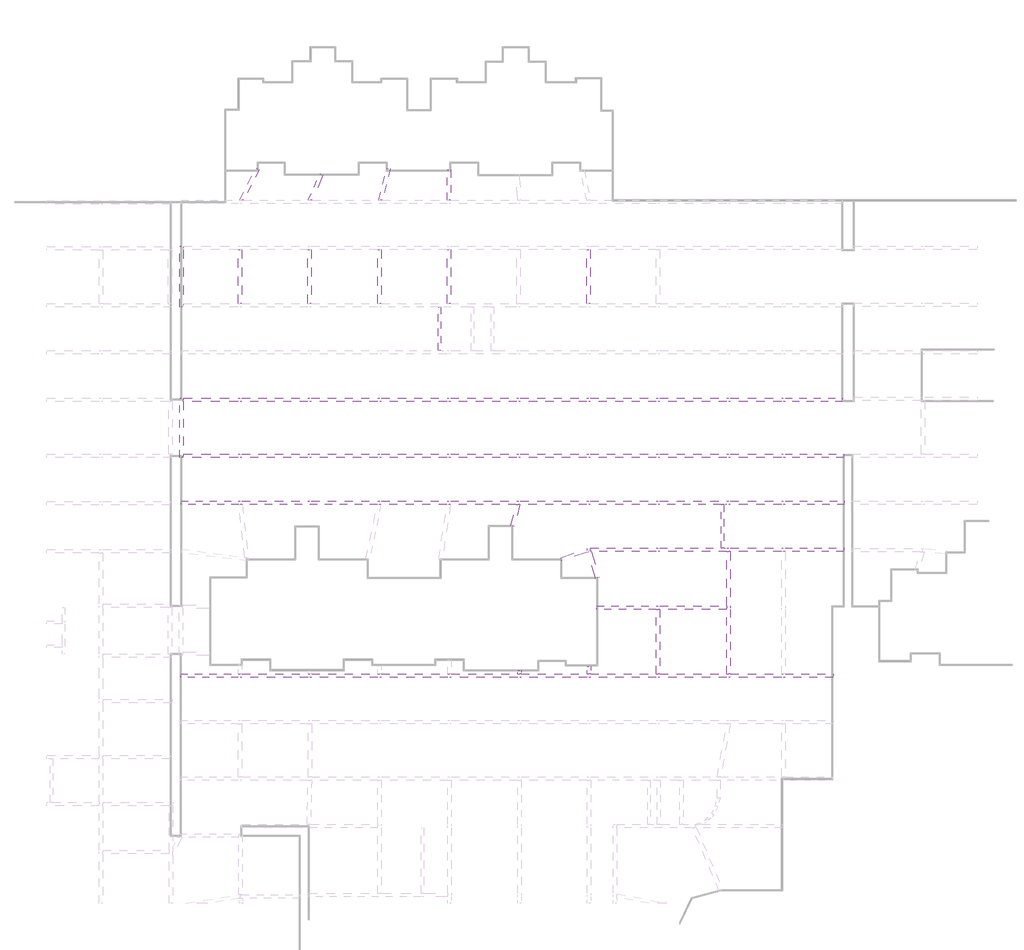
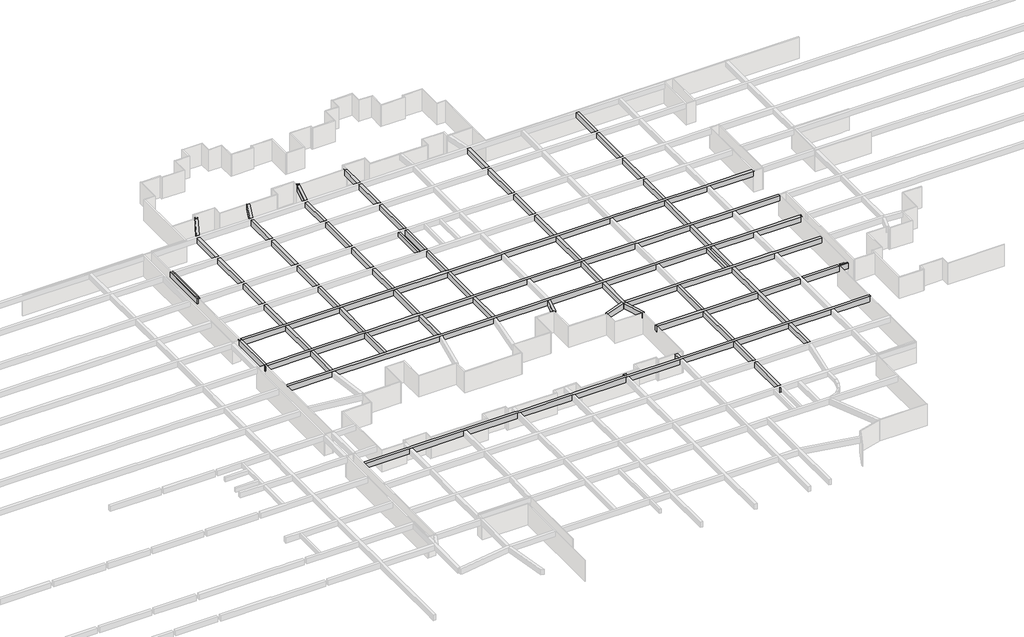
# One storey, part 13 of 16: 26 beams.
"""IFC4 building model written with IfcOpenShell, lengths in millimetres."""

from ifc_helpers import new_model, si_unit, frame, origin, place, context, project, spatial, polyline, outline, extrude, faceted_brep, element, save

model = new_model("IFC4")

# Units and contexts
model_context = context("Model", 3, world=origin())
ifc_project = project(units=[si_unit("LENGTHUNIT", "METRE", prefix="MILLI")], contexts=[model_context])

# Site, building, storey
site = spatial("IfcSite", under=ifc_project)
building = spatial("IfcBuilding", under=site)
storey = spatial("IfcBuildingStorey", under=building, Name="户型图", Elevation=0.0)

# Beams
placement = place(None, origin())
element("IfcBeam", 1, ObjectType="混凝土 - 矩形梁 : KL_beam", at=placement, inside=storey, context=model_context, shape_type="Brep", body=[
    faceted_brep([(256403.757676, -154958.1403142, 3300.0), (256003.757676, -154958.1403142, 3300.0), (256003.757676, -161826.0461868, 3300.0), (256403.757676, -161826.0461868, 3300.0), (256403.757676, -161426.0461868, 3300.0), (256403.757676, -155358.1403142, 3300.0), (256003.757676, -154958.1403142, 2500.0), (256003.757676, -161826.0461868, 2500.0), (256403.757676, -154958.1403142, 2500.0), (256403.757676, -155358.1403142, 2500.0), (256403.757676, -161426.0461868, 2500.0), (256403.757676, -161826.0461868, 2500.0)], [[[0, 1, 2, 3, 4, 5]], [[1, 6, 7, 2]], [[6, 8, 9, 10, 11, 7]], [[8, 0, 5, 4, 3, 11, 10, 9]], [[1, 0, 8, 6]], [[3, 2, 7, 11]]]),
])
element("IfcBeam", 2, ObjectType="混凝土 - 矩形梁 : KL_beam", at=placement, inside=storey, context=model_context, shape_type="Brep", body=[
    faceted_brep([(256403.757676, -137565.7214763, 3300.0), (256003.757676, -137565.7214763, 3300.0), (256003.757676, -144525.7214763, 3300.0), (256403.757676, -144525.7214763, 3300.0), (256403.757676, -144125.7214763, 3300.0), (256403.757676, -137965.7214763, 3300.0), (256403.757676, -137565.7214763, 2500.0), (256403.757676, -144525.7214763, 2500.0), (256403.757676, -144125.7214763, 2500.0), (256403.757676, -137965.7214763, 2500.0), (256003.757676, -137565.7214763, 2500.0), (256003.757676, -144525.7214763, 2500.0)], [[[0, 1, 2, 3, 4, 5]], [[6, 0, 5, 4, 3, 7, 8, 9]], [[10, 6, 9, 8, 7, 11]], [[1, 10, 11, 2]], [[1, 0, 6, 10]], [[3, 2, 11, 7]]]),
])
element("IfcBeam", 3, ObjectType="混凝土 - 矩形梁 : KL_beam", at=placement, inside=storey, context=model_context, shape_type="SweptSolid", body=[
    extrude(outline(polyline([(264780.5419955, -128606.5045486), (265136.9446052, -128788.1007485), (263349.1220942, -132296.8999905), (262900.1915992, -132296.8999905), (264780.5419955, -128606.5045486)])), frame((0.0, 0.0, 2500.0), z_axis=(0.0, 0.0, 1.0), x_axis=(1.0, 0.0, 0.0)), (0.0, 0.0, 1.0), 800.0),
])
element("IfcBeam", 4, ObjectType="混凝土 - 矩形梁 : KL_beam", at=placement, inside=storey, context=model_context, shape_type="SweptSolid", body=[
    extrude(outline(polyline([(272073.9960379, -129262.0850118), (272442.1979793, -129418.3774632), (271220.3376586, -132296.8999905), (270785.7935076, -132296.8999905), (272073.9960379, -129262.0850118)])), frame((0.0, 0.0, 2500.0), z_axis=(0.0, 0.0, 1.0), x_axis=(1.0, 0.0, 0.0)), (0.0, 0.0, 1.0), 800.0),
])
element("IfcBeam", 5, ObjectType="混凝土 - 矩形梁 : KL_beam", at=placement, inside=storey, context=model_context, shape_type="SweptSolid", body=[
    extrude(outline(polyline([(279764.8192397, -128598.9265902), (280152.9375302, -128695.6953484), (279255.0563689, -132296.8999905), (278842.8109172, -132296.8999905), (279764.8192397, -128598.9265902)])), frame((0.0, 0.0, 2500.0), z_axis=(0.0, 0.0, 1.0), x_axis=(1.0, 0.0, 0.0)), (0.0, 0.0, 1.0), 800.0),
])
element("IfcBeam", 6, ObjectType="混凝土 - 矩形梁 : KL_beam", at=placement, inside=storey, context=model_context, shape_type="SweptSolid", body=[
    extrude(outline(polyline([(286699.7203632, -128796.8999905), (287099.7203632, -128796.8999905), (287099.7203632, -132296.8999905), (286699.7203632, -132296.8999905), (286699.7203632, -128796.8999905)])), frame((0.0, 0.0, 2500.0), z_axis=(0.0, 0.0, 1.0), x_axis=(1.0, 0.0, 0.0)), (0.0, 0.0, 1.0), 800.0),
])
element("IfcBeam", 7, ObjectType="混凝土 - 矩形梁 : KL_beam", at=placement, inside=storey, context=model_context, shape_type="Brep", body=[
    faceted_brep([(332003.757676, -154958.1403142, 3300.0), (332003.757676, -155358.1403142, 3300.0), (332003.757676, -155358.1403142, 2500.0), (332003.757676, -154958.1403142, 2500.0), (325452.9173169, -154958.1403142, 3300.0), (325052.9173169, -154958.1403142, 3300.0), (319175.2880408, -154958.1403142, 3300.0), (318775.2880408, -154958.1403142, 3300.0), (311075.2880408, -154958.1403142, 3300.0), (310675.2880408, -154958.1403142, 3300.0), (303119.0558962, -154958.1403142, 3300.0), (302719.0558962, -154958.1403142, 3300.0), (295091.573786, -154958.1403142, 3300.0), (294691.573786, -154958.1403142, 3300.0), (287099.7203632, -154958.1403142, 3300.0), (286699.7203632, -154958.1403142, 3300.0), (279139.6845219, -154958.1403142, 3300.0), (278739.6845219, -154958.1403142, 3300.0), (271118.1706199, -154958.1403142, 3300.0), (270718.1706199, -154958.1403142, 3300.0), (263155.329592, -154958.1403142, 3300.0), (262755.329592, -154958.1403142, 3300.0), (256403.757676, -154958.1403142, 3300.0), (256403.757676, -155358.1403142, 3300.0), (262755.329592, -155358.1403142, 3300.0), (263155.329592, -155358.1403142, 3300.0), (270718.1706199, -155358.1403142, 3300.0), (271118.1706199, -155358.1403142, 3300.0), (278739.6845219, -155358.1403142, 3300.0), (279139.6845219, -155358.1403142, 3300.0), (286699.7203632, -155358.1403142, 3300.0), (287099.7203632, -155358.1403142, 3300.0), (294691.573786, -155358.1403142, 3300.0), (295091.573786, -155358.1403142, 3300.0), (302719.0558962, -155358.1403142, 3300.0), (303119.0558962, -155358.1403142, 3300.0), (310675.2880408, -155358.1403142, 3300.0), (311075.2880408, -155358.1403142, 3300.0), (318775.2880408, -155358.1403142, 3300.0), (319175.2880408, -155358.1403142, 3300.0), (325052.9173169, -155358.1403142, 3300.0), (325452.9173169, -155358.1403142, 3300.0), (256403.757676, -155358.1403142, 2500.0), (262755.329592, -155358.1403142, 2500.0), (263155.329592, -155358.1403142, 2500.0), (270718.1706199, -155358.1403142, 2500.0), (271118.1706199, -155358.1403142, 2500.0), (278739.6845219, -155358.1403142, 2500.0), (279139.6845219, -155358.1403142, 2500.0), (286699.7203632, -155358.1403142, 2500.0), (287099.7203632, -155358.1403142, 2500.0), (294691.573786, -155358.1403142, 2500.0), (295091.573786, -155358.1403142, 2500.0), (302719.0558962, -155358.1403142, 2500.0), (303119.0558962, -155358.1403142, 2500.0), (310675.2880408, -155358.1403142, 2500.0), (311075.2880408, -155358.1403142, 2500.0), (318775.2880408, -155358.1403142, 2500.0), (319175.2880408, -155358.1403142, 2500.0), (325052.9173169, -155358.1403142, 2500.0), (325452.9173169, -155358.1403142, 2500.0), (256403.757676, -154958.1403142, 2500.0), (262755.329592, -154958.1403142, 2500.0), (263155.329592, -154958.1403142, 2500.0), (270718.1706199, -154958.1403142, 2500.0), (271118.1706199, -154958.1403142, 2500.0), (278739.6845219, -154958.1403142, 2500.0), (279139.6845219, -154958.1403142, 2500.0), (286699.7203632, -154958.1403142, 2500.0), (287099.7203632, -154958.1403142, 2500.0), (294691.573786, -154958.1403142, 2500.0), (295091.573786, -154958.1403142, 2500.0), (302719.0558962, -154958.1403142, 2500.0), (303119.0558962, -154958.1403142, 2500.0), (310675.2880408, -154958.1403142, 2500.0), (311075.2880408, -154958.1403142, 2500.0), (318775.2880408, -154958.1403142, 2500.0), (319175.2880408, -154958.1403142, 2500.0), (325052.9173169, -154958.1403142, 2500.0), (325452.9173169, -154958.1403142, 2500.0)], [[[0, 1, 2, 3]], [[1, 0, 4, 5, 6, 7, 8, 9, 10, 11, 12, 13, 14, 15, 16, 17, 18, 19, 20, 21, 22, 23, 24, 25, 26, 27, 28, 29, 30, 31, 32, 33, 34, 35, 36, 37, 38, 39, 40, 41]], [[2, 1, 41, 40, 39, 38, 37, 36, 35, 34, 33, 32, 31, 30, 29, 28, 27, 26, 25, 24, 23, 42, 43, 44, 45, 46, 47, 48, 49, 50, 51, 52, 53, 54, 55, 56, 57, 58, 59, 60]], [[3, 2, 60, 59, 58, 57, 56, 55, 54, 53, 52, 51, 50, 49, 48, 47, 46, 45, 44, 43, 42, 61, 62, 63, 64, 65, 66, 67, 68, 69, 70, 71, 72, 73, 74, 75, 76, 77, 78, 79]], [[0, 3, 79, 78, 77, 76, 75, 74, 73, 72, 71, 70, 69, 68, 67, 66, 65, 64, 63, 62, 61, 22, 21, 20, 19, 18, 17, 16, 15, 14, 13, 12, 11, 10, 9, 8, 7, 6, 5, 4]], [[23, 22, 61, 42]]]),
])
element("IfcBeam", 8, ObjectType="混凝土 - 矩形梁 : KL_beam", at=placement, inside=storey, context=model_context, shape_type="Brep", body=[
    faceted_brep([(332153.7576761, -161426.0461868, 3300.0), (332153.7576761, -161826.0461868, 3300.0), (332153.7576761, -161826.0461868, 2500.0), (332153.7576761, -161426.0461868, 2500.0), (325452.9173169, -161426.0461868, 3300.0), (325052.9173169, -161426.0461868, 3300.0), (319175.2880408, -161426.0461868, 3300.0), (318775.2880408, -161426.0461868, 3300.0), (311075.2880408, -161426.0461868, 3300.0), (310675.2880408, -161426.0461868, 3300.0), (303119.0558962, -161426.0461868, 3300.0), (302719.0558962, -161426.0461868, 3300.0), (295091.573786, -161426.0461868, 3300.0), (294691.573786, -161426.0461868, 3300.0), (287099.7203632, -161426.0461868, 3300.0), (286699.7203632, -161426.0461868, 3300.0), (279139.6845219, -161426.0461868, 3300.0), (278739.6845219, -161426.0461868, 3300.0), (271118.1706199, -161426.0461868, 3300.0), (270718.1706199, -161426.0461868, 3300.0), (263155.329592, -161426.0461868, 3300.0), (262755.329592, -161426.0461868, 3300.0), (256403.757676, -161426.0461868, 3300.0), (256403.757676, -161826.0461868, 3300.0), (262755.329592, -161826.0461868, 3300.0), (263155.329592, -161826.0461868, 3300.0), (270718.1706199, -161826.0461868, 3300.0), (271118.1706199, -161826.0461868, 3300.0), (278739.6845219, -161826.0461868, 3300.0), (279139.6845219, -161826.0461868, 3300.0), (286699.7203632, -161826.0461868, 3300.0), (287099.7203632, -161826.0461868, 3300.0), (294691.573786, -161826.0461868, 3300.0), (295091.573786, -161826.0461868, 3300.0), (302719.0558962, -161826.0461868, 3300.0), (303119.0558962, -161826.0461868, 3300.0), (310675.2880408, -161826.0461868, 3300.0), (311075.2880408, -161826.0461868, 3300.0), (318775.2880408, -161826.0461868, 3300.0), (319175.2880408, -161826.0461868, 3300.0), (325052.9173169, -161826.0461868, 3300.0), (325452.9173169, -161826.0461868, 3300.0), (256403.757676, -161826.0461868, 2500.0), (262755.329592, -161826.0461868, 2500.0), (263155.329592, -161826.0461868, 2500.0), (270718.1706199, -161826.0461868, 2500.0), (271118.1706199, -161826.0461868, 2500.0), (278739.6845219, -161826.0461868, 2500.0), (279139.6845219, -161826.0461868, 2500.0), (286699.7203632, -161826.0461868, 2500.0), (287099.7203632, -161826.0461868, 2500.0), (294691.573786, -161826.0461868, 2500.0), (295091.573786, -161826.0461868, 2500.0), (302719.0558962, -161826.0461868, 2500.0), (303119.0558962, -161826.0461868, 2500.0), (310675.2880408, -161826.0461868, 2500.0), (311075.2880408, -161826.0461868, 2500.0), (318775.2880408, -161826.0461868, 2500.0), (319175.2880408, -161826.0461868, 2500.0), (325052.9173169, -161826.0461868, 2500.0), (325452.9173169, -161826.0461868, 2500.0), (256403.757676, -161426.0461868, 2500.0), (262755.329592, -161426.0461868, 2500.0), (263155.329592, -161426.0461868, 2500.0), (270718.1706199, -161426.0461868, 2500.0), (271118.1706199, -161426.0461868, 2500.0), (278739.6845219, -161426.0461868, 2500.0), (279139.6845219, -161426.0461868, 2500.0), (286699.7203632, -161426.0461868, 2500.0), (287099.7203632, -161426.0461868, 2500.0), (294691.573786, -161426.0461868, 2500.0), (295091.573786, -161426.0461868, 2500.0), (302719.0558962, -161426.0461868, 2500.0), (303119.0558962, -161426.0461868, 2500.0), (310675.2880408, -161426.0461868, 2500.0), (311075.2880408, -161426.0461868, 2500.0), (318775.2880408, -161426.0461868, 2500.0), (319175.2880408, -161426.0461868, 2500.0), (325052.9173169, -161426.0461868, 2500.0), (325452.9173169, -161426.0461868, 2500.0)], [[[0, 1, 2, 3]], [[1, 0, 4, 5, 6, 7, 8, 9, 10, 11, 12, 13, 14, 15, 16, 17, 18, 19, 20, 21, 22, 23, 24, 25, 26, 27, 28, 29, 30, 31, 32, 33, 34, 35, 36, 37, 38, 39, 40, 41]], [[2, 1, 41, 40, 39, 38, 37, 36, 35, 34, 33, 32, 31, 30, 29, 28, 27, 26, 25, 24, 23, 42, 43, 44, 45, 46, 47, 48, 49, 50, 51, 52, 53, 54, 55, 56, 57, 58, 59, 60]], [[3, 2, 60, 59, 58, 57, 56, 55, 54, 53, 52, 51, 50, 49, 48, 47, 46, 45, 44, 43, 42, 61, 62, 63, 64, 65, 66, 67, 68, 69, 70, 71, 72, 73, 74, 75, 76, 77, 78, 79]], [[0, 3, 79, 78, 77, 76, 75, 74, 73, 72, 71, 70, 69, 68, 67, 66, 65, 64, 63, 62, 61, 22, 21, 20, 19, 18, 17, 16, 15, 14, 13, 12, 11, 10, 9, 8, 7, 6, 5, 4]], [[23, 22, 61, 42]]]),
])
element("IfcBeam", 9, ObjectType="混凝土 - 矩形梁 : KL_beam", at=placement, inside=storey, context=model_context, shape_type="Brep", body=[
    faceted_brep([(332253.7576761, -166823.3600959, 3300.0), (332253.7576761, -167223.3600959, 3300.0), (332253.7576761, -167223.3600959, 2500.0), (332253.7576761, -166823.3600959, 2500.0), (256203.7576761, -166823.3600959, 3300.0), (256203.7576761, -166823.3600959, 2500.0), (256203.7576761, -167223.3600959, 2500.0), (256203.7576761, -167223.3600959, 3300.0), (325452.9173169, -166823.3600959, 3300.0), (325052.9173169, -166823.3600959, 3300.0), (319175.2880408, -166823.3600959, 3300.0), (318775.2880408, -166823.3600959, 3300.0), (311075.2880408, -166823.3600959, 3300.0), (310675.2880408, -166823.3600959, 3300.0), (303119.0558962, -166823.3600959, 3300.0), (302719.0558962, -166823.3600959, 3300.0), (295091.573786, -166823.3600959, 3300.0), (294691.573786, -166823.3600959, 3300.0), (287099.7203632, -166823.3600959, 3300.0), (286699.7203632, -166823.3600959, 3300.0), (279139.6845219, -166823.3600959, 3300.0), (278739.6845219, -166823.3600959, 3300.0), (271118.1706199, -166823.3600959, 3300.0), (270718.1706199, -166823.3600959, 3300.0), (263155.329592, -166823.3600959, 3300.0), (262755.329592, -166823.3600959, 3300.0), (262777.848794, -167223.3600959, 3300.0), (263180.706086, -167223.3600959, 3300.0), (278692.7050906, -167223.3600959, 3300.0), (279101.6413286, -167223.3600959, 3300.0), (286667.5284745, -167223.3600959, 3300.0), (287071.9916696, -167223.3600959, 3300.0), (294630.9287114, -167223.3600959, 3300.0), (295045.0391836, -167223.3600959, 3300.0), (302719.0558962, -167223.3600959, 3300.0), (303119.0558962, -167223.3600959, 3300.0), (310675.2880408, -167223.3600959, 3300.0), (311075.2880408, -167223.3600959, 3300.0), (318103.757676, -167223.3600959, 3300.0), (318403.757676, -167223.3600959, 3300.0), (318775.2880408, -167223.3600959, 3300.0), (319175.2880408, -167223.3600959, 3300.0), (325052.9173169, -167223.3600959, 3300.0), (325452.9173169, -167223.3600959, 3300.0), (262777.848794, -167223.3600959, 2500.0), (263180.706086, -167223.3600959, 2500.0), (278692.7050906, -167223.3600959, 2500.0), (279101.6413286, -167223.3600959, 2500.0), (286667.5284745, -167223.3600959, 2500.0), (287071.9916696, -167223.3600959, 2500.0), (294630.9287114, -167223.3600959, 2500.0), (295045.0391836, -167223.3600959, 2500.0), (302719.0558962, -167223.3600959, 2500.0), (303119.0558962, -167223.3600959, 2500.0), (310675.2880408, -167223.3600959, 2500.0), (311075.2880408, -167223.3600959, 2500.0), (318775.2880408, -167223.3600959, 2500.0), (319175.2880408, -167223.3600959, 2500.0), (325052.9173169, -167223.3600959, 2500.0), (325452.9173169, -167223.3600959, 2500.0), (262755.329592, -166823.3600959, 2500.0), (263155.329592, -166823.3600959, 2500.0), (270718.1706199, -166823.3600959, 2500.0), (271118.1706199, -166823.3600959, 2500.0), (278739.6845219, -166823.3600959, 2500.0), (279139.6845219, -166823.3600959, 2500.0), (286699.7203632, -166823.3600959, 2500.0), (287099.7203632, -166823.3600959, 2500.0), (294691.573786, -166823.3600959, 2500.0), (295091.573786, -166823.3600959, 2500.0), (302719.0558962, -166823.3600959, 2500.0), (303119.0558962, -166823.3600959, 2500.0), (310675.2880408, -166823.3600959, 2500.0), (311075.2880408, -166823.3600959, 2500.0), (318775.2880408, -166823.3600959, 2500.0), (319175.2880408, -166823.3600959, 2500.0), (325052.9173169, -166823.3600959, 2500.0), (325452.9173169, -166823.3600959, 2500.0)], [[[0, 1, 2, 3]], [[4, 5, 6, 7]], [[1, 0, 8, 9, 10, 11, 12, 13, 14, 15, 16, 17, 18, 19, 20, 21, 22, 23, 24, 25, 4, 7, 26, 27, 28, 29, 30, 31, 32, 33, 34, 35, 36, 37, 38, 39, 40, 41, 42, 43]], [[2, 1, 43, 42, 41, 40, 39, 38, 37, 36, 35, 34, 33, 32, 31, 30, 29, 28, 27, 26, 7, 6, 44, 45, 46, 47, 48, 49, 50, 51, 52, 53, 54, 55, 56, 57, 58, 59]], [[3, 2, 59, 58, 57, 56, 55, 54, 53, 52, 51, 50, 49, 48, 47, 46, 45, 44, 6, 5, 60, 61, 62, 63, 64, 65, 66, 67, 68, 69, 70, 71, 72, 73, 74, 75, 76, 77]], [[0, 3, 77, 76, 75, 74, 73, 72, 71, 70, 69, 68, 67, 66, 65, 64, 63, 62, 61, 60, 5, 4, 25, 24, 23, 22, 21, 20, 19, 18, 17, 16, 15, 14, 13, 12, 11, 10, 9, 8]]]),
])
element("IfcBeam", 10, ObjectType="混凝土 - 矩形梁 : KL_beam", at=placement, inside=storey, context=model_context, shape_type="Brep", body=[
    faceted_brep([(330953.597965, -186662.1668684, 3300.0), (330953.597965, -187062.1668684, 3300.0), (330953.597965, -187062.1668684, 2500.0), (330953.597965, -186662.1668684, 2500.0), (256118.597965, -186662.1668684, 3300.0), (256118.597965, -186662.1668684, 2500.0), (256118.597965, -187062.1668684, 2500.0), (256118.597965, -187062.1668684, 3300.0), (325452.9173169, -186662.1668684, 3300.0), (325052.9173169, -186662.1668684, 3300.0), (319175.2880408, -186662.1668684, 3300.0), (318775.2880408, -186662.1668684, 3300.0), (311075.2880408, -186662.1668684, 3300.0), (310675.2880408, -186662.1668684, 3300.0), (303155.2880408, -186662.1668684, 3300.0), (302755.2880408, -186662.1668684, 3300.0), (295188.9093069, -186662.1668684, 3300.0), (294788.9093069, -186662.1668684, 3300.0), (287188.9093069, -186662.1668684, 3300.0), (286788.9093069, -186662.1668684, 3300.0), (279139.4840766, -186662.1668684, 3300.0), (278739.4840766, -186662.1668684, 3300.0), (271154.6470805, -186662.1668684, 3300.0), (270754.6470805, -186662.1668684, 3300.0), (263153.757676, -186662.1668684, 3300.0), (262753.757676, -186662.1668684, 3300.0), (262753.757676, -187062.1668684, 3300.0), (263153.757676, -187062.1668684, 3300.0), (270754.6470805, -187062.1668684, 3300.0), (271154.6470805, -187062.1668684, 3300.0), (278739.4840766, -187062.1668684, 3300.0), (279139.4840766, -187062.1668684, 3300.0), (286788.9093069, -187062.1668684, 3300.0), (287188.9093069, -187062.1668684, 3300.0), (294788.9093069, -187062.1668684, 3300.0), (295188.9093069, -187062.1668684, 3300.0), (302755.2880408, -187062.1668684, 3300.0), (303155.2880408, -187062.1668684, 3300.0), (310675.2880408, -187062.1668684, 3300.0), (311075.2880408, -187062.1668684, 3300.0), (318775.2880408, -187062.1668684, 3300.0), (319175.2880408, -187062.1668684, 3300.0), (325052.9173169, -187062.1668684, 3300.0), (325452.9173169, -187062.1668684, 3300.0), (262753.757676, -187062.1668684, 2500.0), (263153.757676, -187062.1668684, 2500.0), (270754.6470805, -187062.1668684, 2500.0), (271154.6470805, -187062.1668684, 2500.0), (278739.4840766, -187062.1668684, 2500.0), (279139.4840766, -187062.1668684, 2500.0), (286788.9093069, -187062.1668684, 2500.0), (287188.9093069, -187062.1668684, 2500.0), (294788.9093069, -187062.1668684, 2500.0), (295188.9093069, -187062.1668684, 2500.0), (302755.2880408, -187062.1668684, 2500.0), (303155.2880408, -187062.1668684, 2500.0), (310675.2880408, -187062.1668684, 2500.0), (311075.2880408, -187062.1668684, 2500.0), (318775.2880408, -187062.1668684, 2500.0), (319175.2880408, -187062.1668684, 2500.0), (325052.9173169, -187062.1668684, 2500.0), (325452.9173169, -187062.1668684, 2500.0), (262753.757676, -186662.1668684, 2500.0), (263153.757676, -186662.1668684, 2500.0), (270754.6470805, -186662.1668684, 2500.0), (271154.6470805, -186662.1668684, 2500.0), (278739.4840766, -186662.1668684, 2500.0), (279139.4840766, -186662.1668684, 2500.0), (286788.9093069, -186662.1668684, 2500.0), (287188.9093069, -186662.1668684, 2500.0), (294788.9093069, -186662.1668684, 2500.0), (295188.9093069, -186662.1668684, 2500.0), (302755.2880408, -186662.1668684, 2500.0), (303155.2880408, -186662.1668684, 2500.0), (310675.2880408, -186662.1668684, 2500.0), (311075.2880408, -186662.1668684, 2500.0), (318775.2880408, -186662.1668684, 2500.0), (319175.2880408, -186662.1668684, 2500.0), (325052.9173169, -186662.1668684, 2500.0), (325452.9173169, -186662.1668684, 2500.0)], [[[0, 1, 2, 3]], [[4, 5, 6, 7]], [[1, 0, 8, 9, 10, 11, 12, 13, 14, 15, 16, 17, 18, 19, 20, 21, 22, 23, 24, 25, 4, 7, 26, 27, 28, 29, 30, 31, 32, 33, 34, 35, 36, 37, 38, 39, 40, 41, 42, 43]], [[2, 1, 43, 42, 41, 40, 39, 38, 37, 36, 35, 34, 33, 32, 31, 30, 29, 28, 27, 26, 7, 6, 44, 45, 46, 47, 48, 49, 50, 51, 52, 53, 54, 55, 56, 57, 58, 59, 60, 61]], [[3, 2, 61, 60, 59, 58, 57, 56, 55, 54, 53, 52, 51, 50, 49, 48, 47, 46, 45, 44, 6, 5, 62, 63, 64, 65, 66, 67, 68, 69, 70, 71, 72, 73, 74, 75, 76, 77, 78, 79]], [[0, 3, 79, 78, 77, 76, 75, 74, 73, 72, 71, 70, 69, 68, 67, 66, 65, 64, 63, 62, 5, 4, 25, 24, 23, 22, 21, 20, 19, 18, 17, 16, 15, 14, 13, 12, 11, 10, 9, 8]]]),
])
element("IfcBeam", 11, ObjectType="混凝土 - 矩形梁 : KL_beam", at=placement, inside=storey, context=model_context, shape_type="SweptSolid", body=[
    extrude(outline(polyline([(302755.2880408, -185762.1668684), (303155.2880408, -185762.1668684), (303155.2880408, -186662.1668684), (302755.2880408, -186662.1668684), (302755.2880408, -185762.1668684)])), frame((0.0, 0.0, 2500.0), z_axis=(0.0, 0.0, 1.0), x_axis=(1.0, 0.0, 0.0)), (0.0, 0.0, 1.0), 800.0),
])
element("IfcBeam", 12, ObjectType="混凝土 - 矩形梁 : KL_beam", at=placement, inside=storey, context=model_context, shape_type="SweptSolid", body=[
    extrude(outline(polyline([(294788.9093069, -186227.0533069), (295188.9093069, -186227.0533069), (295188.9093069, -186662.1668684), (294788.9093069, -186662.1668684), (294788.9093069, -186227.0533069)])), frame((0.0, 0.0, 2500.0), z_axis=(0.0, 0.0, 1.0), x_axis=(1.0, 0.0, 0.0)), (0.0, 0.0, 1.0), 800.0),
])
element("IfcBeam", 13, ObjectType="混凝土 - 矩形梁 : KL_beam", at=placement, inside=storey, context=model_context, shape_type="SweptSolid", body=[
    extrude(outline(polyline([(263155.329592, -166823.3600959), (262755.329592, -166823.3600959), (262755.329592, -161826.0461868), (263155.329592, -161826.0461868), (263155.329592, -166823.3600959)])), frame((0.0, 0.0, 2500.0), z_axis=(0.0, 0.0, 1.0), x_axis=(1.0, 0.0, 0.0)), (0.0, 0.0, 1.0), 800.0),
    extrude(outline(polyline([(262755.329592, -132696.8999905), (263155.329592, -132696.8999905), (263155.329592, -137565.7214763), (262755.329592, -137565.7214763), (262755.329592, -132696.8999905)])), frame((0.0, 0.0, 2500.0), z_axis=(0.0, 0.0, 1.0), x_axis=(1.0, 0.0, 0.0)), (0.0, 0.0, 1.0), 800.0),
    extrude(outline(polyline([(262755.329592, -137965.7214763), (263155.329592, -137965.7214763), (263155.329592, -144125.7214763), (262755.329592, -144125.7214763), (262755.329592, -137965.7214763)])), frame((0.0, 0.0, 2500.0), z_axis=(0.0, 0.0, 1.0), x_axis=(1.0, 0.0, 0.0)), (0.0, 0.0, 1.0), 800.0),
    extrude(outline(polyline([(262755.329592, -144525.7214763), (263155.329592, -144525.7214763), (263155.329592, -149525.7214763), (262755.329592, -149525.7214763), (262755.329592, -144525.7214763)])), frame((0.0, 0.0, 2500.0), z_axis=(0.0, 0.0, 1.0), x_axis=(1.0, 0.0, 0.0)), (0.0, 0.0, 1.0), 800.0),
    extrude(outline(polyline([(262755.329592, -149925.7214763), (263155.329592, -149925.7214763), (263155.329592, -154958.1403142), (262755.329592, -154958.1403142), (262755.329592, -149925.7214763)])), frame((0.0, 0.0, 2500.0), z_axis=(0.0, 0.0, 1.0), x_axis=(1.0, 0.0, 0.0)), (0.0, 0.0, 1.0), 800.0),
    extrude(outline(polyline([(262755.329592, -155358.1403142), (263155.329592, -155358.1403142), (263155.329592, -161426.0461868), (262755.329592, -161426.0461868), (262755.329592, -155358.1403142)])), frame((0.0, 0.0, 2500.0), z_axis=(0.0, 0.0, 1.0), x_axis=(1.0, 0.0, 0.0)), (0.0, 0.0, 1.0), 800.0),
])
element("IfcBeam", 14, ObjectType="混凝土 - 矩形梁 : KL_beam", at=placement, inside=storey, context=model_context, shape_type="SweptSolid", body=[
    extrude(outline(polyline([(270718.1706199, -132696.8999905), (271118.1706199, -132696.8999905), (271118.1706199, -137565.7214763), (270718.1706199, -137565.7214763), (270718.1706199, -132696.8999905)])), frame((0.0, 0.0, 2500.0), z_axis=(0.0, 0.0, 1.0), x_axis=(1.0, 0.0, 0.0)), (0.0, 0.0, 1.0), 800.0),
    extrude(outline(polyline([(271118.1706199, -166823.3600959), (270718.1706199, -166823.3600959), (270718.1706199, -161826.0461868), (271118.1706199, -161826.0461868), (271118.1706199, -166823.3600959)])), frame((0.0, 0.0, 2500.0), z_axis=(0.0, 0.0, 1.0), x_axis=(1.0, 0.0, 0.0)), (0.0, 0.0, 1.0), 800.0),
    extrude(outline(polyline([(270718.1706199, -137965.7214763), (271118.1706199, -137965.7214763), (271118.1706199, -144125.7214763), (270718.1706199, -144125.7214763), (270718.1706199, -137965.7214763)])), frame((0.0, 0.0, 2500.0), z_axis=(0.0, 0.0, 1.0), x_axis=(1.0, 0.0, 0.0)), (0.0, 0.0, 1.0), 800.0),
    extrude(outline(polyline([(270718.1706199, -144525.7214763), (271118.1706199, -144525.7214763), (271118.1706199, -149525.7214763), (270718.1706199, -149525.7214763), (270718.1706199, -144525.7214763)])), frame((0.0, 0.0, 2500.0), z_axis=(0.0, 0.0, 1.0), x_axis=(1.0, 0.0, 0.0)), (0.0, 0.0, 1.0), 800.0),
    extrude(outline(polyline([(270718.1706199, -149925.7214763), (271118.1706199, -149925.7214763), (271118.1706199, -154958.1403142), (270718.1706199, -154958.1403142), (270718.1706199, -149925.7214763)])), frame((0.0, 0.0, 2500.0), z_axis=(0.0, 0.0, 1.0), x_axis=(1.0, 0.0, 0.0)), (0.0, 0.0, 1.0), 800.0),
    extrude(outline(polyline([(270718.1706199, -155358.1403142), (271118.1706199, -155358.1403142), (271118.1706199, -161426.0461868), (270718.1706199, -161426.0461868), (270718.1706199, -155358.1403142)])), frame((0.0, 0.0, 2500.0), z_axis=(0.0, 0.0, 1.0), x_axis=(1.0, 0.0, 0.0)), (0.0, 0.0, 1.0), 800.0),
])
element("IfcBeam", 15, ObjectType="混凝土 - 矩形梁 : KL_beam", at=placement, inside=storey, context=model_context, shape_type="SweptSolid", body=[
    extrude(outline(polyline([(278739.6845219, -132735.2171892), (279139.6845219, -132735.2171892), (279139.6845219, -137565.7214763), (278739.6845219, -137565.7214763), (278739.6845219, -132735.2171892)])), frame((0.0, 0.0, 2500.0), z_axis=(0.0, 0.0, 1.0), x_axis=(1.0, 0.0, 0.0)), (0.0, 0.0, 1.0), 800.0),
    extrude(outline(polyline([(279139.6845219, -166823.3600959), (278739.6845219, -166823.3600959), (278739.6845219, -161826.0461868), (279139.6845219, -161826.0461868), (279139.6845219, -166823.3600959)])), frame((0.0, 0.0, 2500.0), z_axis=(0.0, 0.0, 1.0), x_axis=(1.0, 0.0, 0.0)), (0.0, 0.0, 1.0), 800.0),
    extrude(outline(polyline([(278739.6845219, -137965.7214763), (279139.6845219, -137965.7214763), (279139.6845219, -144125.7214763), (278739.6845219, -144125.7214763), (278739.6845219, -137965.7214763)])), frame((0.0, 0.0, 2500.0), z_axis=(0.0, 0.0, 1.0), x_axis=(1.0, 0.0, 0.0)), (0.0, 0.0, 1.0), 800.0),
    extrude(outline(polyline([(278739.6845219, -144525.7214763), (279139.6845219, -144525.7214763), (279139.6845219, -149525.7214763), (278739.6845219, -149525.7214763), (278739.6845219, -144525.7214763)])), frame((0.0, 0.0, 2500.0), z_axis=(0.0, 0.0, 1.0), x_axis=(1.0, 0.0, 0.0)), (0.0, 0.0, 1.0), 800.0),
    extrude(outline(polyline([(278739.6845219, -149925.7214763), (279139.6845219, -149925.7214763), (279139.6845219, -154958.1403142), (278739.6845219, -154958.1403142), (278739.6845219, -149925.7214763)])), frame((0.0, 0.0, 2500.0), z_axis=(0.0, 0.0, 1.0), x_axis=(1.0, 0.0, 0.0)), (0.0, 0.0, 1.0), 800.0),
    extrude(outline(polyline([(278739.6845219, -155358.1403142), (279139.6845219, -155358.1403142), (279139.6845219, -161426.0461868), (278739.6845219, -161426.0461868), (278739.6845219, -155358.1403142)])), frame((0.0, 0.0, 2500.0), z_axis=(0.0, 0.0, 1.0), x_axis=(1.0, 0.0, 0.0)), (0.0, 0.0, 1.0), 800.0),
])
element("IfcBeam", 16, ObjectType="混凝土 - 矩形梁 : KL_beam", at=placement, inside=storey, context=model_context, shape_type="SweptSolid", body=[
    extrude(outline(polyline([(286699.7203632, -132696.8999905), (287099.7203632, -132696.8999905), (287099.7203632, -137565.7214763), (286699.7203632, -137565.7214763), (286699.7203632, -132696.8999905)])), frame((0.0, 0.0, 2500.0), z_axis=(0.0, 0.0, 1.0), x_axis=(1.0, 0.0, 0.0)), (0.0, 0.0, 1.0), 800.0),
    extrude(outline(polyline([(287099.7203632, -166823.3600959), (286699.7203632, -166823.3600959), (286699.7203632, -161826.0461868), (287099.7203632, -161826.0461868), (287099.7203632, -166823.3600959)])), frame((0.0, 0.0, 2500.0), z_axis=(0.0, 0.0, 1.0), x_axis=(1.0, 0.0, 0.0)), (0.0, 0.0, 1.0), 800.0),
    extrude(outline(polyline([(286699.7203632, -137965.7214763), (287099.7203632, -137965.7214763), (287099.7203632, -144125.7214763), (286699.7203632, -144125.7214763), (286699.7203632, -137965.7214763)])), frame((0.0, 0.0, 2500.0), z_axis=(0.0, 0.0, 1.0), x_axis=(1.0, 0.0, 0.0)), (0.0, 0.0, 1.0), 800.0),
    extrude(outline(polyline([(286699.7203632, -144525.7214763), (287099.7203632, -144525.7214763), (287099.7203632, -149525.7214763), (286699.7203632, -149525.7214763), (286699.7203632, -144525.7214763)])), frame((0.0, 0.0, 2500.0), z_axis=(0.0, 0.0, 1.0), x_axis=(1.0, 0.0, 0.0)), (0.0, 0.0, 1.0), 800.0),
    extrude(outline(polyline([(286699.7203632, -149925.7214763), (287099.7203632, -149925.7214763), (287099.7203632, -154958.1403142), (286699.7203632, -154958.1403142), (286699.7203632, -149925.7214763)])), frame((0.0, 0.0, 2500.0), z_axis=(0.0, 0.0, 1.0), x_axis=(1.0, 0.0, 0.0)), (0.0, 0.0, 1.0), 800.0),
    extrude(outline(polyline([(286699.7203632, -155358.1403142), (287099.7203632, -155358.1403142), (287099.7203632, -161426.0461868), (286699.7203632, -161426.0461868), (286699.7203632, -155358.1403142)])), frame((0.0, 0.0, 2500.0), z_axis=(0.0, 0.0, 1.0), x_axis=(1.0, 0.0, 0.0)), (0.0, 0.0, 1.0), 800.0),
])
element("IfcBeam", 17, ObjectType="混凝土 - 矩形梁 : KL_beam", at=placement, inside=storey, context=model_context, shape_type="SweptSolid", body=[
    extrude(outline(polyline([(294372.1221097, -169734.7208048), (293985.7517792, -169631.1931867), (294630.9287114, -167223.3600959), (295045.0391836, -167223.3600959), (294372.1221097, -169734.7208048)])), frame((0.0, 0.0, 2500.0), z_axis=(0.0, 0.0, 1.0), x_axis=(1.0, 0.0, 0.0)), (0.0, 0.0, 1.0), 800.0),
])
element("IfcBeam", 18, ObjectType="混凝土 - 矩形梁 : KL_beam", at=placement, inside=storey, context=model_context, shape_type="Brep", body=[
    faceted_brep([(303119.0558962, -132696.8999905, 3300.0), (302719.0558962, -132696.8999905, 3300.0), (302719.0558962, -137565.7214763, 3300.0), (303119.0558962, -137565.7214763, 3300.0), (302719.0558962, -132696.8999905, 2500.0), (302719.0558962, -137565.7214763, 2500.0), (303119.0558962, -132696.8999905, 2500.0), (303119.0558962, -137565.7214763, 2500.0)], [[[0, 1, 2, 3]], [[1, 4, 5, 2]], [[4, 6, 7, 5]], [[6, 0, 3, 7]], [[1, 0, 6, 4]], [[3, 2, 5, 7]]]),
    faceted_brep([(302719.0558962, -137965.7214763, 3300.0), (303119.0558962, -137965.7214763, 3300.0), (303119.0558962, -137965.7214763, 2500.0), (302719.0558962, -137965.7214763, 2500.0), (303119.0558962, -144125.7214763, 3300.0), (302719.0558962, -144125.7214763, 3300.0), (302719.0558962, -144125.7214763, 2500.0), (303119.0558962, -144125.7214763, 2500.0)], [[[0, 1, 2, 3]], [[4, 5, 6, 7]], [[1, 0, 5, 4]], [[0, 3, 6, 5]], [[3, 2, 7, 6]], [[2, 1, 4, 7]]]),
    faceted_brep([(303119.0558962, -149525.7214763, 3300.0), (303119.0558962, -144525.7214763, 3300.0), (302719.0558962, -144525.7214763, 3300.0), (302719.0558962, -149525.7214763, 3300.0), (302719.0558962, -144525.7214763, 2500.0), (302719.0558962, -149525.7214763, 2500.0), (303119.0558962, -144525.7214763, 2500.0), (303119.0558962, -149525.7214763, 2500.0)], [[[0, 1, 2, 3]], [[3, 2, 4, 5]], [[5, 4, 6, 7]], [[1, 0, 7, 6]], [[2, 1, 6, 4]], [[0, 3, 5, 7]]]),
    faceted_brep([(302719.0558962, -149925.7214763, 3300.0), (303119.0558962, -149925.7214763, 3300.0), (303119.0558962, -149925.7214763, 2500.0), (302719.0558962, -149925.7214763, 2500.0), (303119.0558962, -154958.1403142, 3300.0), (302719.0558962, -154958.1403142, 3300.0), (302719.0558962, -154958.1403142, 2500.0), (303119.0558962, -154958.1403142, 2500.0)], [[[0, 1, 2, 3]], [[4, 5, 6, 7]], [[4, 1, 0, 5]], [[5, 0, 3, 6]], [[6, 3, 2, 7]], [[1, 4, 7, 2]]]),
    faceted_brep([(302719.0558962, -155358.1403142, 3300.0), (303119.0558962, -155358.1403142, 3300.0), (303119.0558962, -155358.1403142, 2500.0), (302719.0558962, -155358.1403142, 2500.0), (303119.0558962, -161426.0461868, 3300.0), (302719.0558962, -161426.0461868, 3300.0), (302719.0558962, -161426.0461868, 2500.0), (303119.0558962, -161426.0461868, 2500.0)], [[[0, 1, 2, 3]], [[4, 5, 6, 7]], [[4, 1, 0, 5]], [[5, 0, 3, 6]], [[6, 3, 2, 7]], [[1, 4, 7, 2]]]),
    faceted_brep([(302719.0558962, -161826.0461868, 3300.0), (303119.0558962, -161826.0461868, 3300.0), (303119.0558962, -161826.0461868, 2500.0), (302719.0558962, -161826.0461868, 2500.0), (303119.0558962, -166823.3600959, 3300.0), (302719.0558962, -166823.3600959, 3300.0), (302719.0558962, -166823.3600959, 2500.0), (303119.0558962, -166823.3600959, 2500.0)], [[[0, 1, 2, 3]], [[4, 5, 6, 7]], [[1, 0, 5, 4]], [[0, 3, 6, 5]], [[3, 2, 7, 6]], [[2, 1, 4, 7]]]),
    faceted_brep([(302719.0558962, -167223.3600959, 3300.0), (303119.0558962, -167223.3600959, 3300.0), (303119.0558962, -167223.3600959, 2500.0), (302719.0558962, -167223.3600959, 2500.0), (303119.0558962, -172538.8049532, 3300.0), (302788.8440028, -172654.3575143, 3300.0), (302719.0558962, -172678.7787863, 3300.0), (302719.0558962, -172678.7787863, 2500.0), (302788.8440028, -172654.3575143, 2500.0), (303119.0558962, -172538.8049532, 2500.0), (303119.0558962, -172366.9093122, 3300.0), (303119.0558962, -172196.8999905, 3300.0), (302719.0558962, -172254.9950278, 3300.0), (302719.0558962, -172254.9950278, 2500.0), (303119.0558962, -172196.8999905, 2500.0), (303119.0558962, -172366.9093122, 2500.0)], [[[0, 1, 2, 3]], [[4, 5, 6, 7, 8, 9]], [[6, 5, 4, 10, 11, 1, 0, 12]], [[7, 6, 12, 0, 3, 13]], [[9, 8, 7, 13, 3, 2, 14, 15]], [[4, 9, 15, 14, 2, 1, 11, 10]]]),
])
element("IfcBeam", 19, ObjectType="混凝土 - 矩形梁 : KL_beam", at=placement, inside=storey, context=model_context, shape_type="SweptSolid", body=[
    extrude(outline(polyline([(299821.7641207, -173692.6413748), (299689.645954, -173315.0903318), (302719.0558962, -172254.9950278), (302719.0558962, -172678.7787863), (299821.7641207, -173692.6413748)])), frame((0.0, 0.0, 2500.0), z_axis=(0.0, 0.0, 1.0), x_axis=(1.0, 0.0, 0.0)), (0.0, 0.0, 1.0), 800.0),
])
element("IfcBeam", 20, ObjectType="混凝土 - 矩形梁 : KL_beam", at=placement, inside=storey, context=model_context, shape_type="Brep", body=[
    faceted_brep([(304106.4180804, -175585.1104123, 3300.0), (303724.0112948, -175702.4349633, 3300.0), (303724.0112948, -175702.4349633, 2500.0), (304106.4180804, -175585.1104123, 2500.0), (303189.6183289, -172596.8999905, 3300.0), (303119.0558962, -172366.9093122, 3300.0), (303119.0558962, -172538.8049532, 3300.0), (302788.8440028, -172654.3575143, 3300.0), (302788.8440028, -172654.3575143, 2500.0), (303119.0558962, -172538.8049532, 2500.0), (303119.0558962, -172366.9093122, 2500.0), (303189.6183289, -172596.8999905, 2500.0)], [[[0, 1, 2, 3]], [[1, 0, 4, 5, 6, 7]], [[2, 1, 7, 8]], [[3, 2, 8, 9, 10, 11]], [[0, 3, 11, 10, 5, 4]], [[9, 6, 5, 10]], [[6, 9, 8, 7]]]),
])
element("IfcBeam", 21, ObjectType="混凝土 - 矩形梁 : KL_beam", at=placement, inside=storey, context=model_context, shape_type="Brep", body=[
    faceted_brep([(332153.4067861, -172196.8999905, 3300.0), (332153.4067861, -172596.8999905, 3300.0), (332153.4067861, -172596.8999905, 2500.0), (332153.4067861, -172196.8999905, 2500.0), (325452.9173169, -172196.8999905, 3300.0), (325052.9173169, -172196.8999905, 3300.0), (319175.2880408, -172196.8999905, 3300.0), (318775.2880408, -172196.8999905, 3300.0), (318403.757676, -172196.8999905, 3300.0), (318103.757676, -172196.8999905, 3300.0), (311075.2880408, -172196.8999905, 3300.0), (310675.2880408, -172196.8999905, 3300.0), (303119.0558962, -172196.8999905, 3300.0), (303119.0558962, -172366.9093122, 3300.0), (303189.6183289, -172596.8999905, 3300.0), (310675.2880408, -172596.8999905, 3300.0), (311075.2880408, -172596.8999905, 3300.0), (318775.2880408, -172596.8999905, 3300.0), (319175.2880408, -172596.8999905, 3300.0), (325052.9173169, -172596.8999905, 3300.0), (325452.9173169, -172596.8999905, 3300.0), (303189.6183289, -172596.8999905, 2500.0), (310675.2880408, -172596.8999905, 2500.0), (311075.2880408, -172596.8999905, 2500.0), (318775.2880408, -172596.8999905, 2500.0), (319175.2880408, -172596.8999905, 2500.0), (325052.9173169, -172596.8999905, 2500.0), (325452.9173169, -172596.8999905, 2500.0), (303119.0558962, -172366.9093122, 2500.0), (303119.0558962, -172196.8999905, 2500.0), (310675.2880408, -172196.8999905, 2500.0), (311075.2880408, -172196.8999905, 2500.0), (318775.2880408, -172196.8999905, 2500.0), (319175.2880408, -172196.8999905, 2500.0), (325052.9173169, -172196.8999905, 2500.0), (325452.9173169, -172196.8999905, 2500.0)], [[[0, 1, 2, 3]], [[1, 0, 4, 5, 6, 7, 8, 9, 10, 11, 12, 13, 14, 15, 16, 17, 18, 19, 20]], [[2, 1, 20, 19, 18, 17, 16, 15, 14, 21, 22, 23, 24, 25, 26, 27]], [[3, 2, 27, 26, 25, 24, 23, 22, 21, 28, 29, 30, 31, 32, 33, 34, 35]], [[0, 3, 35, 34, 33, 32, 31, 30, 29, 12, 11, 10, 9, 8, 7, 6, 5, 4]], [[12, 29, 28, 13]], [[14, 13, 28, 21]]]),
])
element("IfcBeam", 22, ObjectType="混凝土 - 矩形梁 : KL_beam", at=placement, inside=storey, context=model_context, shape_type="Brep", body=[
    faceted_brep([(319175.2880408, -132696.8999905, 3300.0), (318775.2880408, -132696.8999905, 3300.0), (318775.2880408, -137565.7214763, 3300.0), (319175.2880408, -137565.7214763, 3300.0), (318775.2880408, -132696.8999905, 2500.0), (318775.2880408, -137565.7214763, 2500.0), (319175.2880408, -132696.8999905, 2500.0), (319175.2880408, -137565.7214763, 2500.0)], [[[0, 1, 2, 3]], [[1, 4, 5, 2]], [[4, 6, 7, 5]], [[6, 0, 3, 7]], [[1, 0, 6, 4]], [[3, 2, 5, 7]]]),
    faceted_brep([(319175.2880408, -191962.1668684, 3300.0), (318775.2880408, -191962.1668684, 3300.0), (318775.2880408, -191962.1668684, 2500.0), (319175.2880408, -191962.1668684, 2500.0), (318775.2880408, -187062.1668684, 3300.0), (319175.2880408, -187062.1668684, 3300.0), (319175.2880408, -187062.1668684, 2500.0), (318775.2880408, -187062.1668684, 2500.0)], [[[0, 1, 2, 3]], [[4, 5, 6, 7]], [[1, 0, 5, 4]], [[2, 1, 4, 7]], [[3, 2, 7, 6]], [[0, 3, 6, 5]]]),
    faceted_brep([(318775.2880408, -137965.7214763, 3300.0), (319175.2880408, -137965.7214763, 3300.0), (319175.2880408, -137965.7214763, 2500.0), (318775.2880408, -137965.7214763, 2500.0), (319175.2880408, -144125.7214763, 3300.0), (318775.2880408, -144125.7214763, 3300.0), (318775.2880408, -144125.7214763, 2500.0), (319175.2880408, -144125.7214763, 2500.0)], [[[0, 1, 2, 3]], [[4, 5, 6, 7]], [[1, 0, 5, 4]], [[0, 3, 6, 5]], [[3, 2, 7, 6]], [[2, 1, 4, 7]]]),
    faceted_brep([(319175.2880408, -144525.7214763, 3300.0), (318775.2880408, -144525.7214763, 3300.0), (318775.2880408, -149525.7214763, 3300.0), (319175.2880408, -149525.7214763, 3300.0), (318775.2880408, -144525.7214763, 2500.0), (318775.2880408, -149525.7214763, 2500.0), (319175.2880408, -144525.7214763, 2500.0), (319175.2880408, -149525.7214763, 2500.0)], [[[0, 1, 2, 3]], [[1, 4, 5, 2]], [[4, 6, 7, 5]], [[6, 0, 3, 7]], [[1, 0, 6, 4]], [[3, 2, 5, 7]]]),
    faceted_brep([(318775.2880408, -149925.7214763, 3300.0), (319175.2880408, -149925.7214763, 3300.0), (319175.2880408, -149925.7214763, 2500.0), (318775.2880408, -149925.7214763, 2500.0), (319175.2880408, -154958.1403142, 3300.0), (318775.2880408, -154958.1403142, 3300.0), (318775.2880408, -154958.1403142, 2500.0), (319175.2880408, -154958.1403142, 2500.0)], [[[0, 1, 2, 3]], [[4, 5, 6, 7]], [[1, 0, 5, 4]], [[0, 3, 6, 5]], [[3, 2, 7, 6]], [[2, 1, 4, 7]]]),
    faceted_brep([(319175.2880408, -155358.1403142, 3300.0), (318775.2880408, -155358.1403142, 3300.0), (318775.2880408, -161426.0461868, 3300.0), (319175.2880408, -161426.0461868, 3300.0), (318775.2880408, -155358.1403142, 2500.0), (318775.2880408, -161426.0461868, 2500.0), (319175.2880408, -155358.1403142, 2500.0), (319175.2880408, -161426.0461868, 2500.0)], [[[0, 1, 2, 3]], [[1, 4, 5, 2]], [[4, 6, 7, 5]], [[6, 0, 3, 7]], [[1, 0, 6, 4]], [[3, 2, 5, 7]]]),
    faceted_brep([(318775.2880408, -161826.0461868, 3300.0), (319175.2880408, -161826.0461868, 3300.0), (319175.2880408, -161826.0461868, 2500.0), (318775.2880408, -161826.0461868, 2500.0), (319175.2880408, -166823.3600959, 3300.0), (318775.2880408, -166823.3600959, 3300.0), (318775.2880408, -166823.3600959, 2500.0), (319175.2880408, -166823.3600959, 2500.0)], [[[0, 1, 2, 3]], [[4, 5, 6, 7]], [[1, 0, 5, 4]], [[0, 3, 6, 5]], [[3, 2, 7, 6]], [[2, 1, 4, 7]]]),
    faceted_brep([(319175.2880408, -167223.3600959, 3300.0), (318775.2880408, -167223.3600959, 3300.0), (318775.2880408, -172196.8999905, 3300.0), (319175.2880408, -172196.8999905, 3300.0), (318775.2880408, -167223.3600959, 2500.0), (318775.2880408, -172196.8999905, 2500.0), (319175.2880408, -167223.3600959, 2500.0), (319175.2880408, -172196.8999905, 2500.0)], [[[0, 1, 2, 3]], [[1, 4, 5, 2]], [[4, 6, 7, 5]], [[6, 0, 3, 7]], [[1, 0, 6, 4]], [[3, 2, 5, 7]]]),
    faceted_brep([(319175.2880408, -186662.1668684, 3300.0), (318775.2880408, -186662.1668684, 3300.0), (318775.2880408, -186662.1668684, 2500.0), (319175.2880408, -186662.1668684, 2500.0), (318775.2880408, -172596.8999905, 3300.0), (319175.2880408, -172596.8999905, 3300.0), (319175.2880408, -172596.8999905, 2500.0), (318775.2880408, -172596.8999905, 2500.0), (319175.2880408, -179243.9042946, 3300.0), (319175.2880408, -178843.9042946, 3300.0), (318775.2880408, -178843.9042946, 3300.0), (318775.2880408, -179243.9042946, 3300.0), (318775.2880408, -178843.9042946, 2500.0), (318775.2880408, -179243.9042946, 2500.0), (319175.2880408, -178843.9042946, 2500.0), (319175.2880408, -179243.9042946, 2500.0)], [[[0, 1, 2, 3]], [[4, 5, 6, 7]], [[1, 0, 8, 9, 5, 4, 10, 11]], [[2, 1, 11, 10, 4, 7, 12, 13]], [[3, 2, 13, 12, 7, 6, 14, 15]], [[0, 3, 15, 14, 6, 5, 9, 8]]]),
])
element("IfcBeam", 23, ObjectType="混凝土 - 矩形梁 : KL_beam", at=placement, inside=storey, context=model_context, shape_type="Brep", body=[
    faceted_brep([(332153.7053404, -178843.9042946, 3300.0), (332153.7053404, -179243.9042946, 3300.0), (332153.7053404, -179243.9042946, 2500.0), (332153.7053404, -178843.9042946, 2500.0), (325452.9173169, -178843.9042946, 3300.0), (325452.9173169, -179243.9042946, 3300.0), (325452.9173169, -179243.9042946, 2500.0), (325452.9173169, -178843.9042946, 2500.0)], [[[0, 1, 2, 3]], [[1, 0, 4, 5]], [[2, 1, 5, 6]], [[3, 2, 6, 7]], [[0, 3, 7, 4]], [[5, 4, 7, 6]]]),
    faceted_brep([(303822.7053404, -178843.9042946, 3300.0), (303822.7053404, -178843.9042946, 2500.0), (303822.7053404, -179243.9042946, 2500.0), (303822.7053404, -179243.9042946, 3300.0), (318775.2880408, -178843.9042946, 3300.0), (318775.2880408, -179243.9042946, 3300.0), (318775.2880408, -179243.9042946, 2500.0), (318775.2880408, -178843.9042946, 2500.0), (310675.2880408, -179243.9042946, 3300.0), (311075.2880408, -179243.9042946, 3300.0), (311075.2880408, -178843.9042946, 3300.0), (310675.2880408, -178843.9042946, 3300.0), (310675.2880408, -179243.9042946, 2500.0), (311075.2880408, -179243.9042946, 2500.0), (310675.2880408, -178843.9042946, 2500.0), (311075.2880408, -178843.9042946, 2500.0)], [[[0, 1, 2, 3]], [[4, 5, 6, 7]], [[0, 3, 8, 9, 5, 4, 10, 11]], [[3, 2, 12, 13, 6, 5, 9, 8]], [[2, 1, 14, 15, 7, 6, 13, 12]], [[1, 0, 11, 10, 4, 7, 15, 14]]]),
    faceted_brep([(319175.2880408, -179243.9042946, 3300.0), (319175.2880408, -178843.9042946, 3300.0), (319175.2880408, -178843.9042946, 2500.0), (319175.2880408, -179243.9042946, 2500.0), (325052.9173169, -178843.9042946, 3300.0), (325052.9173169, -179243.9042946, 3300.0), (325052.9173169, -179243.9042946, 2500.0), (325052.9173169, -178843.9042946, 2500.0)], [[[0, 1, 2, 3]], [[4, 5, 6, 7]], [[1, 0, 5, 4]], [[0, 3, 6, 5]], [[3, 2, 7, 6]], [[2, 1, 4, 7]]]),
])
element("IfcBeam", 24, ObjectType="混凝土 - 矩形梁 : KL_beam", at=placement, inside=storey, context=model_context, shape_type="Brep", body=[
    faceted_brep([(310675.2880408, -198896.8999905, 3300.0), (310675.2880408, -198896.8999905, 2500.0), (311075.2880408, -198896.8999905, 2500.0), (311075.2880408, -198896.8999905, 2700.0), (310805.2880408, -198896.8999905, 2700.0), (310805.2880408, -198896.8999905, 3300.0), (310675.2880408, -198870.1471774, 3300.0), (310805.2880408, -198870.1471774, 3300.0), (310675.2880408, -198870.1471774, 2500.0), (311075.2880408, -198870.1471774, 2500.0), (311075.2880408, -198870.1471774, 2700.0), (310805.2880408, -198870.1471774, 2700.0)], [[[0, 1, 2, 3, 4, 5]], [[6, 0, 5, 7]], [[1, 0, 6, 8]], [[2, 1, 8, 9]], [[2, 9, 10, 3]], [[8, 6, 7, 11, 10, 9]], [[4, 11, 7, 5]], [[11, 4, 3, 10]]]),
    faceted_brep([(310675.2880408, -172596.8999905, 3300.0), (311075.2880408, -172596.8999905, 3300.0), (311075.2880408, -172596.8999905, 2500.0), (310675.2880408, -172596.8999905, 2500.0), (311075.2880408, -178843.9042946, 3300.0), (310675.2880408, -178843.9042946, 3300.0), (310675.2880408, -178843.9042946, 2500.0), (311075.2880408, -178843.9042946, 2500.0)], [[[0, 1, 2, 3]], [[4, 5, 6, 7]], [[1, 0, 5, 4]], [[0, 3, 6, 5]], [[3, 2, 7, 6]], [[2, 1, 4, 7]]]),
    faceted_brep([(310675.2880408, -187062.1668684, 3300.0), (311075.2880408, -187062.1668684, 3300.0), (311075.2880408, -187062.1668684, 2500.0), (310675.2880408, -187062.1668684, 2500.0), (311075.2880408, -191962.1668684, 3300.0), (310675.2880408, -191962.1668684, 3300.0), (310675.2880408, -191962.1668684, 2500.0), (311075.2880408, -191962.1668684, 2500.0)], [[[0, 1, 2, 3]], [[4, 5, 6, 7]], [[1, 0, 5, 4]], [[0, 3, 6, 5]], [[3, 2, 7, 6]], [[2, 1, 4, 7]]]),
    faceted_brep([(311075.2880408, -186662.1668684, 3300.0), (310675.2880408, -186662.1668684, 3300.0), (310675.2880408, -186662.1668684, 2500.0), (311075.2880408, -186662.1668684, 2500.0), (311075.2880408, -179243.9042946, 3300.0), (310675.2880408, -179243.9042946, 3300.0), (310675.2880408, -179243.9042946, 2500.0), (311075.2880408, -179243.9042946, 2500.0)], [[[0, 1, 2, 3]], [[1, 0, 4, 5]], [[2, 1, 5, 6]], [[3, 2, 6, 7]], [[0, 3, 7, 4]], [[5, 4, 7, 6]]]),
    faceted_brep([(310675.2880408, -192362.1668684, 3300.0), (311075.2880408, -192362.1668684, 3300.0), (311075.2880408, -192362.1668684, 2500.0), (310675.2880408, -192362.1668684, 2500.0), (310675.2880408, -198470.1471774, 3300.0), (310675.2880408, -198470.1471774, 2500.0), (311075.2880408, -198470.1471774, 2500.0), (311075.2880408, -198470.1471774, 2700.0), (311075.2880408, -198470.1471774, 3300.0), (310805.2880408, -198470.1471774, 3300.0)], [[[0, 1, 2, 3]], [[4, 5, 6, 7, 8, 9]], [[1, 0, 4, 9, 8]], [[0, 3, 5, 4]], [[3, 2, 6, 5]], [[2, 1, 8, 7, 6]]]),
])
element("IfcBeam", 25, ObjectType="混凝土 - 矩形梁 : L_beam", at=placement, inside=storey, context=model_context, shape_type="SweptSolid", body=[
    extrude(outline(polyline([(285649.7203632, -144525.7214763), (285949.7203632, -144525.7214763), (285949.7203632, -149525.7214763), (285649.7203632, -149525.7214763), (285649.7203632, -144525.7214763)])), frame((0.0, 0.0, 2700.0), z_axis=(0.0, 0.0, 1.0), x_axis=(1.0, 0.0, 0.0)), (0.0, 0.0, 1.0), 600.0),
])
element("IfcBeam", 26, ObjectType="混凝土 - 矩形梁 : L_beam", at=placement, inside=storey, context=model_context, shape_type="SweptSolid", body=[
    extrude(outline(polyline([(318103.757676, -167223.3600959), (318403.757676, -167223.3600959), (318403.757676, -172196.8999905), (318103.757676, -172196.8999905), (318103.757676, -167223.3600959)])), frame((0.0, 0.0, 2700.0), z_axis=(0.0, 0.0, 1.0), x_axis=(1.0, 0.0, 0.0)), (0.0, 0.0, 1.0), 600.0),
])

save(model, "model.ifc")

# Revit data of these elements
# Type "混凝土 - 矩形梁 : KL_beam"
#   Length [instance default] = 1524 mm
#   b = 400 mm
#   h = 800 mm
#   Structural Material [instance default] = 混凝土 - 现场浇注混凝土
#   Assembly Code = ""
# Type "混凝土 - 矩形梁 : L_beam"
#   Length [instance default] = 1524 mm
#   b = 300 mm
#   h = 600 mm
#   Structural Material [instance default] = none
#   Assembly Code = ""
# Elements 1, 2, 3, 4, 5, 6, 7, 8, 9, 10, 11, 12, 13, 14, 15, 16, 17, 18, 19, 20, 21, 22, 23, 24 (IfcBeam, "混凝土 - 矩形梁 : KL_beam")
#   Comments = ""
#   Structural Material = none
#   Phase Created = 新构造
# Elements 25, 26 (IfcBeam, "混凝土 - 矩形梁 : L_beam")
#   Comments = ""
#   Structural Material = none
#   Phase Created = 新构造
# Materials
#   "混凝土 - 现场浇注混凝土": class "混凝土", colour RGB 192 192 192, transparency 0
